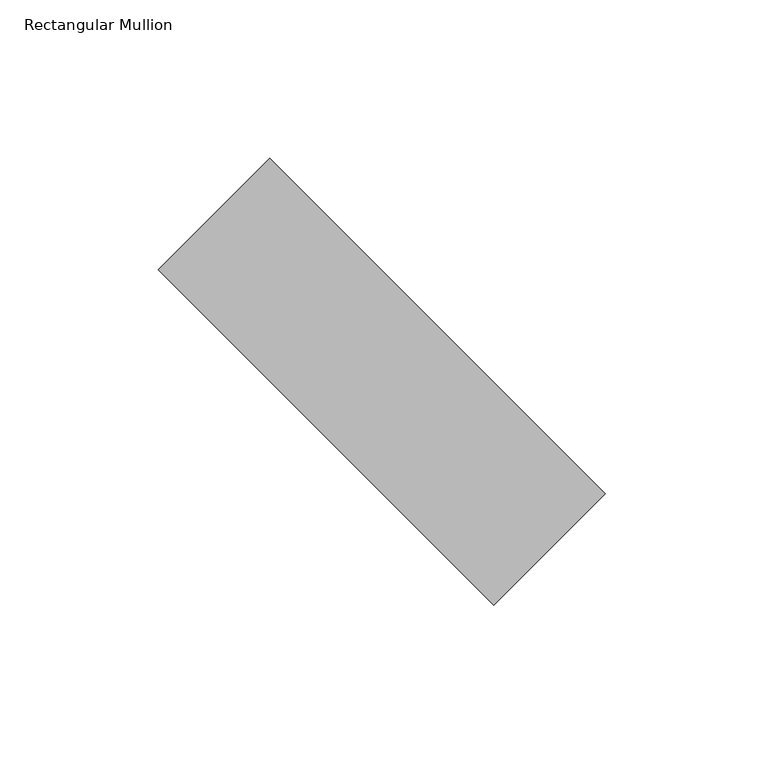
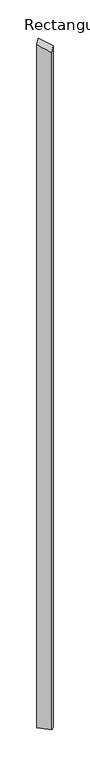
"""IFC4 building model written with IfcOpenShell, lengths in millimetres: member geometry, Rectangular Mullion : tilted mullions."""

from ifc_helpers import new_model, si_unit, origin, place, context, project, spatial, faceted_brep, source, transform, mapped, element, save


def rectangular_mullion_bea0bdf5(model_context):
    return source(origin(), model_context, "Body", "Brep", [
        faceted_brep([(-35.3553391, 70.7106781, -7999.3358332), (70.7106781, -35.3553391, -7999.3358332), (35.3553391, -70.7106781, -7999.3358332), (-70.7106781, 35.3553391, -7999.3358332), (-70.7106781, 35.3553391, 10.0090632), (-35.3553391, 70.7106781, 55.0597182), (35.3553391, -70.7106781, -55.0597182), (70.7106781, -35.3553391, -10.0090632)], [[[0, 1, 2, 3]], [[4, 5, 0, 3]], [[6, 4, 3, 2]], [[7, 6, 2, 1]], [[5, 7, 1, 0]], [[5, 4, 6, 7]]]),
    ])


if __name__ == "__main__":
    model = new_model("IFC4")
    model_context = context("Model", 3, world=origin())
    ifc_project = project(units=[si_unit("LENGTHUNIT", "METRE", prefix="MILLI")], contexts=[model_context])
    site = spatial("IfcSite", under=ifc_project)
    building = spatial("IfcBuilding", under=site)
    placement = place(None, origin())
    rectangular_mullion_shape = rectangular_mullion_bea0bdf5(model_context)
    element("IfcMember", 1, ObjectType="Rectangular Mullion : tilted mullions", at=placement, inside=building, context=model_context, shape_type="MappedRepresentation", body=[
        mapped(rectangular_mullion_shape, transform((0.0, 0.0, 0.0), x_axis=(1.0, 0.0, 0.0), y_axis=(0.0, 1.0, 0.0), z_axis=(0.0, 0.0, 1.0))),
    ])
    save(model, "model.ifc")

# Revit data of these elements
# Type "Rectangular Mullion : tilted mullions"
#   built-in parameter 1007304 = 0.492126 (stored number, unit not read)
#   built-in parameter 1007301 = 0.082021 (stored number, unit not read)
#   built-in parameter 1007300 = 0.082021 (stored number, unit not read)
# Element 1 (IfcMember, "Rectangular Mullion : tilted mullions")
#   Materials on its faces: "Aluminum"
# Materials
#   "Aluminum": class "Metal", colour RGB 244 244 244, transparency 0, Description = "Aluminum 6061", Cost = 0
